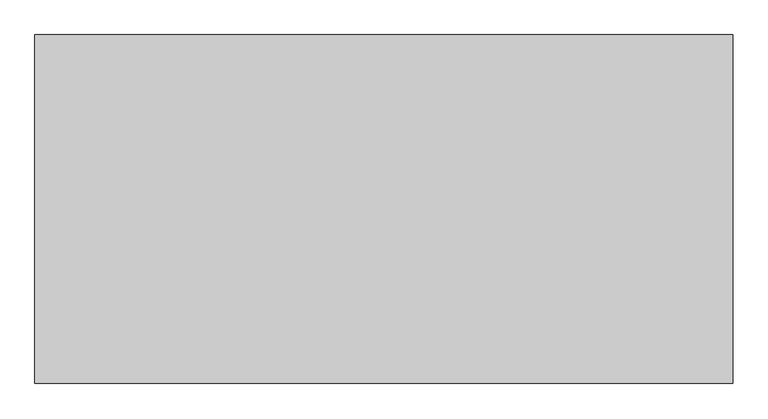
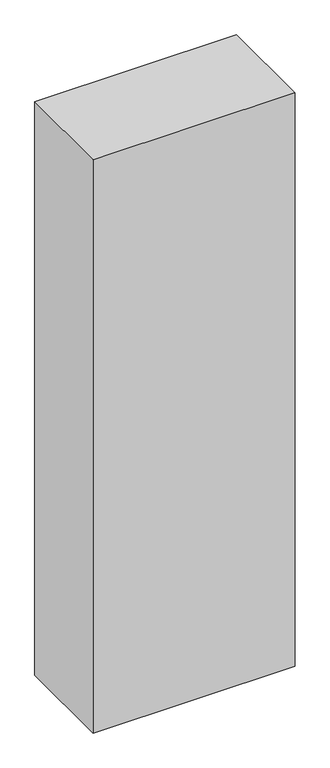
"""IFC4 building model written with IfcOpenShell, lengths in millimetres: proxy geometry, Space Planning Box_hec : Space Planning Box_hec."""

import ifcopenshell
import ifcopenshell.guid

model = None  # the IFC model being written
_history = None  # IfcOwnerHistory: only IFC2X3 demands one
_inside = {}  # id of a spatial element -> (the spatial element, [elements in it])
_under = {}  # id of a project, library or spatial element -> (it, [spatial elements below it])
_declared = {}  # id of a project -> (the project, [libraries it declares])
_typed = {}  # id of a type object -> (the type object, [elements of that type])
_made_of = {}  # id of a material, layer set ... -> (it, [elements and type objects made of it])


def new_model(schema):
    """Start an empty IFC model of exactly this schema.

    Asked for "IFC4X3", IfcOpenShell would pick the latest addendum, in which some entities
    have other attributes; the version numbers below select the first issue.
    IFC2X3 requires an IfcOwnerHistory on every rooted entity: one is made here for all.
    """
    global model, _history
    if schema == "IFC4X3":
        model = ifcopenshell.file(schema_version=(4, 3, 0, 0))
    else:
        model = ifcopenshell.file(schema=schema)
    _inside.clear()
    _under.clear()
    _declared.clear()
    _typed.clear()
    _made_of.clear()
    _history = None
    if model.schema == "IFC2X3":
        org = make("IfcOrganization", Name="unknown")
        user = make(
            "IfcPersonAndOrganization",
            ThePerson=make("IfcPerson", FamilyName="unknown"),
            TheOrganization=org,
        )
        app = make(
            "IfcApplication",
            ApplicationDeveloper=org,
            Version="unknown",
            ApplicationFullName="unknown",
            ApplicationIdentifier="unknown",
        )
        _history = make(
            "IfcOwnerHistory",
            OwningUser=user,
            OwningApplication=app,
            ChangeAction="ADDED",
            CreationDate=0,
        )
    return model


def make(cls, **values):
    """One entity of the class cls with the attributes given. An attribute that is None is left unset."""
    return model.create_entity(
        cls, **{name: value for name, value in values.items() if value is not None}
    )


def rooted(cls, **values):
    """An entity with a GlobalId (a new one), such as an element, a storey or a relation."""
    return make(cls, GlobalId=ifcopenshell.guid.new(), OwnerHistory=_history, **values)


def si_unit(unit_type, name, prefix=None):
    """IfcSIUnit, for example si_unit("LENGTHUNIT", "METRE", prefix="MILLI")."""
    return make("IfcSIUnit", UnitType=unit_type, Prefix=prefix, Name=name)


def assignment(units):
    """IfcUnitAssignment: the units of a project."""
    return None if units is None else make("IfcUnitAssignment", Units=units)


def point(xyz):
    """IfcCartesianPoint."""
    return None if xyz is None else make("IfcCartesianPoint", Coordinates=xyz)


def direction(xyz):
    """IfcDirection."""
    return None if xyz is None else make("IfcDirection", DirectionRatios=xyz)


def frame(location, z_axis=None, x_axis=None):
    """IfcAxis2Placement3D, a coordinate frame: its origin and axes. An axis left out is left unset."""
    return make(
        "IfcAxis2Placement3D",
        Location=point(location),
        Axis=direction(z_axis),
        RefDirection=direction(x_axis),
    )


def origin():
    """The frame at (0, 0, 0) with its axes left unset."""
    return frame((0.0, 0.0, 0.0))


def origin_with_axes():
    """The frame at (0, 0, 0) with the z axis (0, 0, 1) and the x axis (1, 0, 0) written out."""
    return frame((0.0, 0.0, 0.0), z_axis=(0.0, 0.0, 1.0), x_axis=(1.0, 0.0, 0.0))


def place(relative_to, where):
    """IfcLocalPlacement: puts the frame where relative to a parent placement (None: the world)."""
    return make(
        "IfcLocalPlacement", PlacementRelTo=relative_to, RelativePlacement=where
    )


def context(
    kind, dimensions, precision=None, world=None, true_north=None, identifier=None
):
    """IfcGeometricRepresentationContext, for example the 3D "Model" context."""
    return make(
        "IfcGeometricRepresentationContext",
        ContextIdentifier=identifier,
        ContextType=kind,
        CoordinateSpaceDimension=dimensions,
        Precision=precision,
        WorldCoordinateSystem=world,
        TrueNorth=true_north,
    )


def project(units=None, contexts=None):
    """IfcProject with its units and contexts."""
    return rooted(
        "IfcProject",
        Name="project",
        RepresentationContexts=contexts,
        UnitsInContext=assignment(units),
    )


def spatial(cls, under=None, at=None, **own):
    """A site, building, storey or space (cls), placed at a placement, below another one or the project."""
    s = rooted(cls, ObjectPlacement=at, **own)
    if under is not None:
        _under.setdefault(under.id(), (under, []))[1].append(s)
    return s


def polyline(points):
    """IfcPolyline through the points."""
    return make("IfcPolyline", Points=[point(p) for p in points])


def outline(outer, holes=None, kind="AREA"):
    """IfcArbitraryClosedProfileDef: a profile drawn as a closed curve; with holes, ...WithVoids."""
    if holes is None:
        return make("IfcArbitraryClosedProfileDef", ProfileType=kind, OuterCurve=outer)
    return make(
        "IfcArbitraryProfileDefWithVoids",
        ProfileType=kind,
        OuterCurve=outer,
        InnerCurves=holes,
    )


def extrude(swept, where, along, depth):
    """IfcExtrudedAreaSolid: the profile swept, set in the frame where, extruded along a direction by depth."""
    return make(
        "IfcExtrudedAreaSolid",
        SweptArea=swept,
        Position=where,
        ExtrudedDirection=direction(along),
        Depth=depth,
    )


def shape(context_of_items, identifier, shape_type, items):
    """IfcShapeRepresentation: the items that make up one representation, for example the "Body"."""
    return make(
        "IfcShapeRepresentation",
        ContextOfItems=context_of_items,
        RepresentationIdentifier=identifier,
        RepresentationType=shape_type,
        Items=items,
    )


def source(mapping_origin, context_of_items, identifier, shape_type, items):
    """IfcRepresentationMap: a shape defined once, which mapped items show again and again."""
    return make(
        "IfcRepresentationMap",
        MappingOrigin=mapping_origin,
        MappedRepresentation=shape(context_of_items, identifier, shape_type, items),
    )


def transform(
    local_origin,
    x_axis=None,
    y_axis=None,
    z_axis=None,
    scale=None,
    scale2=None,
    scale3=None,
    uniform=True,
):
    """IfcCartesianTransformationOperator3D, or its non-uniform kind. x_axis, y_axis, z_axis: its Axis1, 2, 3."""
    if uniform:
        return make(
            "IfcCartesianTransformationOperator3D",
            Axis1=direction(x_axis),
            Axis2=direction(y_axis),
            LocalOrigin=point(local_origin),
            Scale=scale,
            Axis3=direction(z_axis),
        )
    return make(
        "IfcCartesianTransformationOperator3DnonUniform",
        Axis1=direction(x_axis),
        Axis2=direction(y_axis),
        LocalOrigin=point(local_origin),
        Scale=scale,
        Axis3=direction(z_axis),
        Scale2=scale2,
        Scale3=scale3,
    )


def mapped(mapping_source, mapping_target):
    """IfcMappedItem: shows the shape of a source again, moved by a transform."""
    return make(
        "IfcMappedItem", MappingSource=mapping_source, MappingTarget=mapping_target
    )


def made_of(thing, what):
    """Note that an element or type object is made of a material, layer set ...; save() writes the relation."""
    if what is not None:
        _made_of.setdefault(what.id(), (what, []))[1].append(thing)
    return thing


def element(
    cls,
    number,
    at=None,
    inside=None,
    cuts=None,
    type_object=None,
    material=None,
    context=None,
    identifier="Body",
    shape_type=None,
    held_by="IfcProductDefinitionShape",
    body=None,
    shapes=None,
    **own,
):
    """One element of the class cls, such as IfcWall. Its Tag is "e" and its number.

    at: its placement. inside: the storey or other place that contains it. cuts: it is an
    opening in that element (IfcRelVoidsElement). A single representation is given by context,
    identifier, shape_type and body (its items); several are given by shapes. held_by: the class
    of the entity that holds the representations. save() writes the other relations.
    """
    e = rooted(cls, Tag="e%d" % number, ObjectPlacement=at, **own)
    if body is not None:
        shapes = [shape(context, identifier, shape_type, body)]
    if shapes is not None:
        e.Representation = make(held_by, Representations=shapes)
    if inside is not None:
        _inside.setdefault(inside.id(), (inside, []))[1].append(e)
    if cuts is not None:
        rooted(
            "IfcRelVoidsElement", RelatingBuildingElement=cuts, RelatedOpeningElement=e
        )
    if type_object is not None:
        _typed.setdefault(type_object.id(), (type_object, []))[1].append(e)
    return made_of(e, material)


def aggregate(whole, parts):
    """IfcRelAggregates: a whole, such as a stair, and the parts it consists of."""
    return rooted("IfcRelAggregates", RelatingObject=whole, RelatedObjects=parts)


def save(model, path):
    """Write the relations noted so far, then the file.

    IfcRelAggregates (storeys below a building ...), IfcRelContainedInSpatialStructure (elements
    in a storey), IfcRelDefinesByType, IfcRelAssociatesMaterial and IfcRelDeclares: one each for
    every whole, place, type object, material and project.
    """
    for whole, parts in _under.values():
        aggregate(whole, parts)
    for where, things in _inside.values():
        rooted(
            "IfcRelContainedInSpatialStructure",
            RelatedElements=things,
            RelatingStructure=where,
        )
    for kind, things in _typed.values():
        rooted("IfcRelDefinesByType", RelatedObjects=things, RelatingType=kind)
    for what, things in _made_of.values():
        rooted("IfcRelAssociatesMaterial", RelatedObjects=things, RelatingMaterial=what)
    for by, libraries in _declared.values():
        rooted("IfcRelDeclares", RelatingContext=by, RelatedDefinitions=libraries)
    model.write(path)


def generic_models_da00a96f(model_context):
    return source(origin(), model_context, "Body", "SweptSolid", [
        extrude(outline(polyline([(1000.0, 500.0), (1000.0, -500.0), (-1000.0, -500.0), (-1000.0, 500.0), (1000.0, 500.0)])), origin_with_axes(), (0.0, 0.0, 1.0), 6000.0),
    ])


if __name__ == "__main__":
    model = new_model("IFC4")
    model_context = context("Model", 3, world=origin())
    ifc_project = project(units=[si_unit("LENGTHUNIT", "METRE", prefix="MILLI")], contexts=[model_context])
    site = spatial("IfcSite", under=ifc_project)
    building = spatial("IfcBuilding", under=site)
    placement = place(None, origin())
    generic_models_shape = generic_models_da00a96f(model_context)
    element("IfcBuildingElementProxy", 1, Name="Space Planning Box_hec : Space Planning Box_hec", ObjectType="Space Planning Box_hec : Space Planning Box_hec", at=placement, inside=building, context=model_context, shape_type="MappedRepresentation", body=[
        mapped(generic_models_shape, transform((0.0, 0.0, 0.0), x_axis=(1.0, 0.0, 0.0), y_axis=(0.0, 1.0, 0.0), z_axis=(0.0, 0.0, 1.0))),
    ])
    save(model, "model.ifc")

# Revit data of these elements
# Type "Space Planning Box_hec : Space Planning Box_hec"
#   Type Comments = "..."
#   Room Name [instance default] = "?"
#   Interior Finish [instance default] = ""
#   Exterior Finish [instance default] = ""
#   Department [instance default] = ""
#   Assembly Code = "..."
#   Width [instance default] = 1524 mm
#   Program Area [instance default] = 0.00 m²
#   Length [instance default] = 1524 mm
#   Height [instance default] = 1524 mm
#   Area [instance default] = 2.32258 m²
#   Fill Color [instance default] = Cyan
#   Default Elevation = 0
# Element 1 (IfcBuildingElementProxy, "Space Planning Box_hec : Space Planning Box_hec")
#   Room Name = "Corridor"
#   Interior Finish = "IF2-1"
#   Exterior Finish = "EF1"
#   Department = "AR"
#   Width = 2000 mm
#   Length = 1000 mm
#   Height = 6000 mm
#   Area = 2.00 m²
#   Fill Color = Lavender
#   Materials on its faces: "Lavender"
# Materials
#   "Cyan": class "Generic", colour RGB 0 255 255, transparency 0.2, Cost = 0
#   "Lavender": class "Generic", colour RGB 186 85 211, transparency 0.2, Cost = 0
